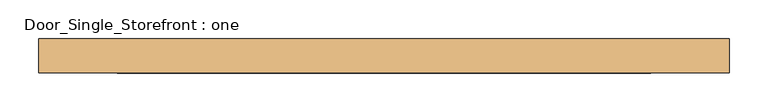
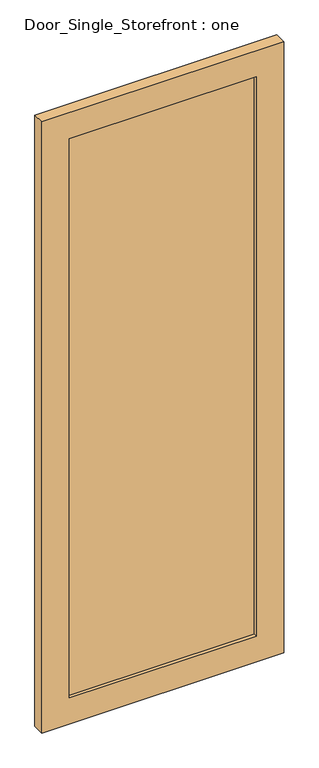
"""IFC4 building model written with IfcOpenShell, lengths in millimetres: door geometry, Door_Single_Storefront : one."""

from ifc_helpers import new_model, si_unit, frame, origin, place, context, project, spatial, polyline, outline, extrude, source, transform, mapped, element, save


def door_single_storefront_one_d4a41a43(model_context):
    return source(origin(), model_context, "Body", "SweptSolid", [
        extrude(outline(polyline([(2387.6, -446.88125), (0.0, -446.88125), (0.0, 446.88125), (2387.6, 446.88125), (2387.6, -446.88125)]), holes=[polyline([(101.6, 345.28125), (101.6, -345.28125), (2286.0, -345.28125), (2286.0, 345.28125), (101.6, 345.28125)])]), frame((0.0, -19.05, 0.0), z_axis=(0.0, 1.0, 0.0), x_axis=(0.0, 0.0, 1.0)), (0.0, 0.0, 1.0), 44.45),
        extrude(outline(polyline([(345.28125, -6.35), (-345.28125, -6.35), (-345.28125, 12.7), (345.28125, 12.7), (345.28125, -6.35)])), frame((0.0, 0.0, 101.6), z_axis=(0.0, 0.0, 1.0), x_axis=(1.0, 0.0, 0.0)), (0.0, 0.0, 1.0), 2184.4),
    ])


if __name__ == "__main__":
    model = new_model("IFC4")
    model_context = context("Model", 3, world=origin())
    ifc_project = project(units=[si_unit("LENGTHUNIT", "METRE", prefix="MILLI")], contexts=[model_context])
    site = spatial("IfcSite", under=ifc_project)
    building = spatial("IfcBuilding", under=site)
    placement = place(None, origin())
    door_single_storefront_one_shape = door_single_storefront_one_d4a41a43(model_context)
    element("IfcDoor", 1, ObjectType="Door_Single_Storefront : one", at=placement, inside=building, context=model_context, shape_type="MappedRepresentation", body=[
        mapped(door_single_storefront_one_shape, transform((0.0, 0.0, 0.0), x_axis=(1.0, 0.0, 0.0), y_axis=(0.0, 1.0, 0.0), z_axis=(0.0, 0.0, 1.0))),
    ])
    save(model, "model.ifc")

# Revit data of these elements
# Type "Door_Single_Storefront : one"
#   Type Mark = "27"
#   Analytic Construction = "<None>"
#   Stile_Width = 0' - 4"
#   Door_Thickness = 0' - 1 3/4"
#   Door_Offset = 0' - 1"
#   Glass_Material = Glass
#   Frame_Material = Aluminum
#   Function = (empty or 0)
# Element 1 (IfcDoor, "Door_Single_Storefront : one")
#   Materials on its faces: "Aluminum", "Glass"
# Materials
#   "Glass": class "Glass", colour RGB 142 168 196, transparency 0.75, Description = "Soda Lime Glass", Cost = 0
#   "Aluminum": class "Metal", colour RGB 226 226 226, transparency 0, Description = "Aluminum 6061", Cost = 0
